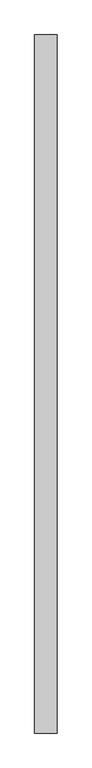
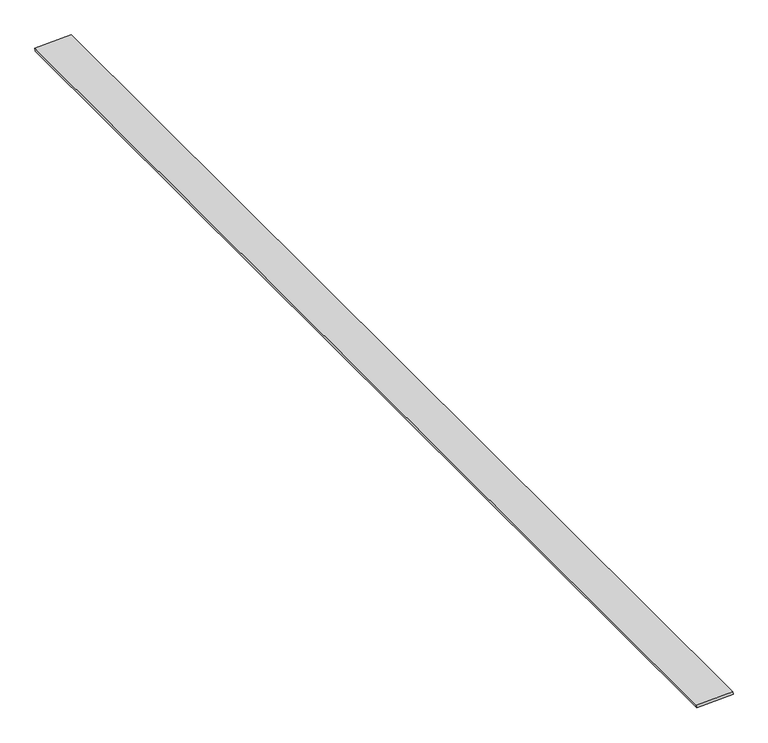
"""IFC4 building model written with IfcOpenShell, lengths in millimetres: proxy geometry, Generic Models 7:Generic Models 1:2:Generic Models 1:2 : Generic Models 7:Generic Models 1:337419:21 : Generic Models 7:Generic Models 1:2:Generic Models 1:2 : Generic Models 7:Generic Models 1:337419:306751."""

from ifc_helpers import new_model, si_unit, frame, origin, place, context, project, spatial, polyline, outline, extrude, source, transform, mapped, element, save


def generic_models_55cb2431(model_context):
    return source(origin(), model_context, "Body", "SweptSolid", [
        extrude(outline(polyline([(3680.0317016, 560598.5553746), (3686.1783289, 560753.9982303), (3698.8684401, 560753.4964293), (3692.3921975, 560598.0666074), (3680.0317016, 560598.5553746)])), frame((0.0, -548060.3163841, 0.0), z_axis=(0.0, 1.0, 0.0), x_axis=(0.0, 0.0, 1.0)), (0.0, 0.0, 1.0), 4876.8),
    ])


if __name__ == "__main__":
    model = new_model("IFC4")
    model_context = context("Model", 3, world=origin())
    ifc_project = project(units=[si_unit("LENGTHUNIT", "METRE", prefix="MILLI")], contexts=[model_context])
    site = spatial("IfcSite", under=ifc_project)
    building = spatial("IfcBuilding", under=site)
    placement = place(None, origin())
    generic_models_shape = generic_models_55cb2431(model_context)
    element("IfcBuildingElementProxy", 1, Name="Generic Models 7:Generic Models 1:2:Generic Models 1:2 : Generic Models 7:Generic Models 1:337419:21 : Generic Models 7:Generic Models 1:2:Generic Models 1:2 : Generic Models 7:Generic Models 1:337419:306751", ObjectType="Generic Models 7:Generic Models 1:2:Generic Models 1:2 : Generic Models 7:Generic Models 1:337419:21 : Generic Models 7:Generic Models 1:2:Generic Models 1:2 : Generic Models 7:Generic Models 1:337419:306751", at=placement, inside=building, context=model_context, shape_type="MappedRepresentation", body=[
        mapped(generic_models_shape, transform((0.0, 0.0, 0.0), x_axis=(1.0, 0.0, 0.0), y_axis=(0.0, 1.0, 0.0), z_axis=(0.0, 0.0, 1.0))),
    ])
    save(model, "model.ifc")

# Revit data of these elements
# Type "Generic Models 7:Generic Models 1:2:Generic Models 1:2 : Generic Models 7:Generic Models 1:337419:21 : Generic Models 7:Generic Models 1:2:Generic Models 1:2 : Generic Models 7:Generic Models 1:337419:306751"
#   NameOverride = "Generic Models 7:Generic Models 1:2:Generic Models 1:2 : Generic Models 7:Generic Models 1:337419:306751"
#   ObjectTypeOverride = "Generic Models 1:2 : Generic Models 7:Generic Models 1:337419"
#   Reference = "Generic Models 1"
#   Tag = "306751"
# Element 1 (IfcBuildingElementProxy, "Generic Models 7:Generic Models 1:2:Generic Models 1:2 : Generic Models 7:Generic Models 1:337419:21 : Generic Models 7:Generic Models 1:2:Generic Models 1:2 : Generic Models 7:Generic Models 1:337419:306751")
#   Materials on its faces: "BLOCKING - SIZE AS NEC."
# Materials
#   "BLOCKING - SIZE AS NEC.": class "Wood", colour RGB 144 113 62, transparency 0, Description = "Pinus Echinata", Cost = 0
